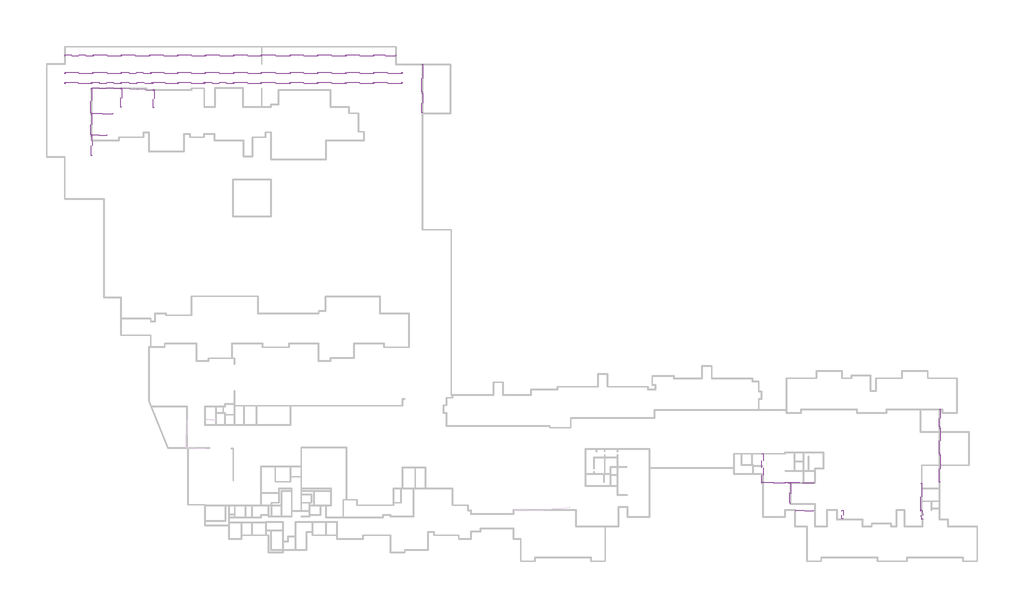
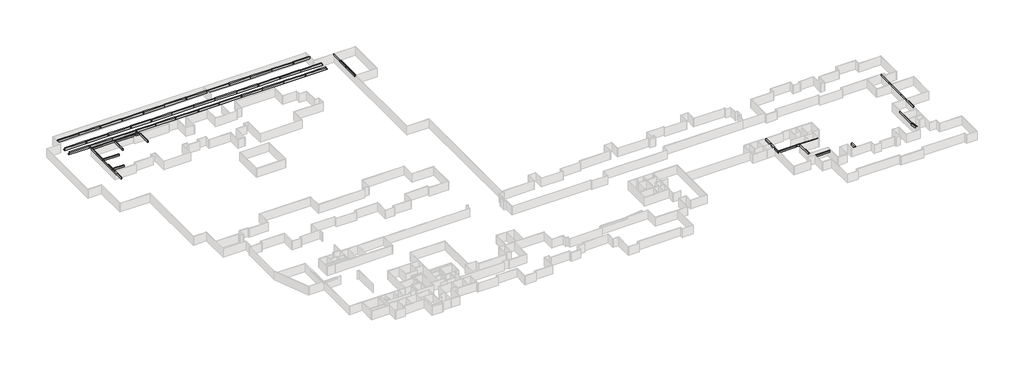
# One storey, part 8 of 8: 58 beams.
"""IFC4 building model written with IfcOpenShell, lengths in millimetres."""

from ifc_helpers import new_model, si_unit, frame, origin, place, context, project, spatial, polyline, outline, extrude, faceted_brep, element, save

model = new_model("IFC4")

# Units and contexts
model_context = context("Model", 3, world=origin())
ifc_project = project(units=[si_unit("LENGTHUNIT", "METRE", prefix="MILLI")], contexts=[model_context])

# Site, building, storey
site = spatial("IfcSite", under=ifc_project)
building = spatial("IfcBuilding", under=site)
storey = spatial("IfcBuildingStorey", under=building, Name="户型图", Elevation=0.0)

# Beams
placement = place(None, origin())
element("IfcBeam", 1, ObjectType="混凝土 - 矩形梁 : KL_beam", at=placement, inside=storey, context=model_context, shape_type="Brep", body=[
    faceted_brep([(69846.6115888, 146493.9951293, 3300.0), (69823.484619, 146214.2806226, 3300.0), (69695.5125279, 146193.9951293, 3300.0), (69833.6976621, 146193.9951293, 3300.0), (77972.7452463, 146193.9951293, 3300.0), (77972.7452463, 146493.9951293, 3300.0), (69695.5125279, 146193.9951293, 2700.0), (69833.6976621, 146193.9951293, 2700.0), (77972.7452463, 146193.9951293, 2700.0), (69823.484619, 146214.2806226, 2700.0), (69846.6115888, 146493.9951293, 2700.0), (77972.7452463, 146493.9951293, 2700.0)], [[[0, 1, 2, 3, 4, 5]], [[2, 6, 7, 8, 4, 3]], [[9, 10, 11, 8, 7, 6]], [[10, 0, 5, 11]], [[9, 1, 0, 10]], [[1, 9, 6, 2]], [[5, 4, 8, 11]]]),
])
element("IfcBeam", 2, ObjectType="混凝土 - 矩形梁 : KL_beam", at=placement, inside=storey, context=model_context, shape_type="SweptSolid", body=[
    extrude(outline(polyline([(69533.6976621, 146168.3450494), (69695.5125279, 146193.9951293), (69833.6976621, 146193.9951293), (69833.6976621, 139317.045189), (69533.6976621, 139317.045189), (69533.6976621, 146168.3450494)])), frame((0.0, 0.0, 2700.0), z_axis=(0.0, 0.0, 1.0), x_axis=(1.0, 0.0, 0.0)), (0.0, 0.0, 1.0), 600.0),
])
element("IfcBeam", 3, ObjectType="混凝土 - 矩形梁 : KL_beam", at=placement, inside=storey, context=model_context, shape_type="SweptSolid", body=[
    extrude(outline(polyline([(75683.6976621, 139317.045189), (75683.6976621, 139017.045189), (69858.8476291, 139017.045189), (69858.8476291, 139317.045189), (75683.6976621, 139317.045189)])), frame((0.0, 0.0, 2700.0), z_axis=(0.0, 0.0, 1.0), x_axis=(1.0, 0.0, 0.0)), (0.0, 0.0, 1.0), 600.0),
])
element("IfcBeam", 4, ObjectType="混凝土 - 矩形梁 : KL_beam", at=placement, inside=storey, context=model_context, shape_type="Brep", body=[
    faceted_brep([(78272.7452463, 140994.6198884, 3300.0), (77972.7452463, 140994.6198884, 3300.0), (77972.7452463, 140994.6198884, 2700.0), (78272.7452463, 140994.6198884, 2700.0), (78272.7452463, 146185.5002249, 3300.0), (78272.7452463, 146193.9951293, 3300.0), (77972.7452463, 146193.9951293, 3300.0), (77972.7452463, 146193.9951293, 2700.0), (78272.7452463, 146193.9951293, 2700.0), (78272.7452463, 146185.5002249, 2700.0)], [[[0, 1, 2, 3]], [[1, 0, 4, 5, 6]], [[2, 1, 6, 7]], [[3, 2, 7, 8, 9]], [[0, 3, 9, 8, 5, 4]], [[6, 5, 8, 7]]]),
])
element("IfcBeam", 5, ObjectType="混凝土 - 矩形梁 : KL_beam", at=placement, inside=storey, context=model_context, shape_type="Brep", body=[
    faceted_brep([(87344.6832098, 140893.8703738, 3300.0), (87044.6832098, 140893.8703738, 3300.0), (87044.6832098, 140893.8703738, 2700.0), (87344.6832098, 140893.8703738, 2700.0), (87344.6832098, 145855.8003854, 3300.0), (87044.6832098, 145832.1898733, 3300.0), (87044.6832098, 145702.0347295, 3300.0), (87044.6832098, 145832.1898733, 2700.0), (87044.6832098, 145702.0347295, 2700.0), (87344.6832098, 145855.8003854, 2700.0)], [[[0, 1, 2, 3]], [[1, 0, 4, 5, 6]], [[2, 1, 6, 5, 7, 8]], [[3, 2, 8, 7, 9]], [[0, 3, 9, 4]], [[4, 9, 7, 5]]]),
])
element("IfcBeam", 6, ObjectType="混凝土 - 矩形梁 : KL_beam", at=placement, inside=storey, context=model_context, shape_type="Brep", body=[
    faceted_brep([(78272.7452463, 146485.9555292, 3300.0), (78272.7452463, 146193.9951293, 3300.0), (78272.7452463, 146185.5002249, 3300.0), (87044.6832098, 145702.0347295, 3300.0), (87044.6832098, 145832.1898733, 3300.0), (87017.4727846, 146003.9897368, 3300.0), (78272.7452463, 146185.5002249, 2700.0), (87044.6832098, 145702.0347295, 2700.0), (78272.7452463, 146193.9951293, 2700.0), (78272.7452463, 146485.9555292, 2700.0), (87017.4727846, 146003.9897368, 2700.0), (87044.6832098, 145832.1898733, 2700.0)], [[[0, 1, 2, 3, 4, 5]], [[2, 6, 7, 3]], [[6, 8, 9, 10, 11, 7]], [[9, 0, 5, 10]], [[0, 9, 8, 6, 2, 1]], [[5, 4, 11, 10]], [[4, 3, 7, 11]]]),
])
element("IfcBeam", 7, ObjectType="混凝土 - 矩形梁 : KL_beam", at=placement, inside=storey, context=model_context, shape_type="Brep", body=[
    faceted_brep([(73982.1511869, 133204.2446453, 3300.0), (73982.1511869, 132904.2446453, 3300.0), (73982.1511869, 132904.2446453, 2700.0), (73982.1511869, 133204.2446453, 2700.0), (69833.6976621, 133204.2446453, 3300.0), (69833.6976621, 132904.2446453, 3300.0), (69835.8783333, 132904.2446453, 3300.0), (69833.6976621, 132904.2446453, 2700.0), (69835.8783333, 132904.2446453, 2700.0), (69833.6976621, 133204.2446453, 2700.0)], [[[0, 1, 2, 3]], [[1, 0, 4, 5, 6]], [[2, 1, 6, 5, 7, 8]], [[3, 2, 8, 7, 9]], [[0, 3, 9, 4]], [[5, 4, 9, 7]]]),
])
element("IfcBeam", 8, ObjectType="混凝土 - 矩形梁 : KL_beam", at=placement, inside=storey, context=model_context, shape_type="Brep", body=[
    faceted_brep([(258434.4881621, 35441.452007, 3300.0), (258434.4881621, 35141.452007, 3300.0), (264873.3530817, 35141.452007, 3300.0), (264873.3530817, 35441.452007, 3300.0), (258734.4881621, 35441.452007, 3300.0), (258434.4881621, 35441.452007, 2700.0), (264873.3530817, 35441.452007, 2700.0), (258734.4881621, 35441.452007, 2700.0), (258434.4881621, 35141.452007, 2700.0), (264873.3530817, 35141.452007, 2700.0)], [[[0, 1, 2, 3, 4]], [[5, 0, 4, 3, 6, 7]], [[8, 5, 7, 6, 9]], [[1, 8, 9, 2]], [[3, 2, 9, 6]], [[1, 0, 5, 8]]]),
])
element("IfcBeam", 9, ObjectType="混凝土 - 矩形梁 : KL_beam", at=placement, inside=storey, context=model_context, shape_type="SweptSolid", body=[
    extrude(outline(polyline([(258434.4881621, 43489.0128116), (258588.4160503, 43497.0798304), (258734.4881621, 43497.0798304), (258734.4881621, 35441.452007), (258434.4881621, 35441.452007), (258434.4881621, 43489.0128116)])), frame((0.0, 0.0, 2700.0), z_axis=(0.0, 0.0, 1.0), x_axis=(1.0, 0.0, 0.0)), (0.0, 0.0, 1.0), 600.0),
])
element("IfcBeam", 10, ObjectType="混凝土 - 矩形梁 : KL_beam", at=placement, inside=storey, context=model_context, shape_type="SweptSolid", body=[
    extrude(outline(polyline([(308273.5691593, 50816.8475615), (308573.5691593, 50816.8475615), (308573.5691593, 43416.8475615), (308273.5691593, 43416.8475615), (308273.5691593, 50816.8475615)])), frame((0.0, 0.0, 2700.0), z_axis=(0.0, 0.0, 1.0), x_axis=(1.0, 0.0, 0.0)), (0.0, 0.0, 1.0), 600.0),
])
element("IfcBeam", 11, ObjectType="混凝土 - 矩形梁 : KL_beam", at=placement, inside=storey, context=model_context, shape_type="SweptSolid", body=[
    extrude(outline(polyline([(308273.5691593, 43116.8475615), (308573.5691593, 43116.8475615), (308573.5691593, 35416.8475615), (308273.5691593, 35416.8475615), (308273.5691593, 43116.8475615)])), frame((0.0, 0.0, 2700.0), z_axis=(0.0, 0.0, 1.0), x_axis=(1.0, 0.0, 0.0)), (0.0, 0.0, 1.0), 600.0),
])
element("IfcBeam", 12, ObjectType="混凝土 - 矩形梁 : KL_beam", at=placement, inside=storey, context=model_context, shape_type="SweptSolid", body=[
    extrude(outline(polyline([(308273.5691593, 55914.1029719), (308573.5691593, 55914.1029719), (308573.5691593, 51116.8475615), (308273.5691593, 51116.8475615), (308273.5691593, 55914.1029719)])), frame((0.0, 0.0, 2700.0), z_axis=(0.0, 0.0, 1.0), x_axis=(1.0, 0.0, 0.0)), (0.0, 0.0, 1.0), 600.0),
])
element("IfcBeam", 13, ObjectType="混凝土 - 矩形梁 : KL_beam", at=placement, inside=storey, context=model_context, shape_type="SweptSolid", body=[
    extrude(outline(polyline([(162705.5468539, 144918.3398855), (163005.5468539, 144918.3398855), (163005.5468539, 139418.3398855), (162705.5468539, 139418.3398855), (162705.5468539, 144918.3398855)])), frame((0.0, 0.0, 2700.0), z_axis=(0.0, 0.0, 1.0), x_axis=(1.0, 0.0, 0.0)), (0.0, 0.0, 1.0), 600.0),
])
element("IfcBeam", 14, ObjectType="混凝土 - 矩形梁 : KL_beam", at=placement, inside=storey, context=model_context, shape_type="SweptSolid", body=[
    extrude(outline(polyline([(162705.5468539, 153068.3398855), (163005.5468539, 153068.3398855), (163005.5468539, 145218.3398855), (162705.5468539, 145218.3398855), (162705.5468539, 153068.3398855)])), frame((0.0, 0.0, 2700.0), z_axis=(0.0, 0.0, 1.0), x_axis=(1.0, 0.0, 0.0)), (0.0, 0.0, 1.0), 600.0),
])
element("IfcBeam", 15, ObjectType="混凝土 - 矩形梁 : KL_beam", at=placement, inside=storey, context=model_context, shape_type="SweptSolid", body=[
    extrude(outline(polyline([(69833.6976621, 133204.2446453), (69533.6976621, 133204.2446453), (69533.6976621, 139017.045189), (69833.6976621, 139017.045189), (69833.6976621, 133204.2446453)])), frame((0.0, 0.0, 2700.0), z_axis=(0.0, 0.0, 1.0), x_axis=(1.0, 0.0, 0.0)), (0.0, 0.0, 1.0), 600.0),
])
element("IfcBeam", 16, ObjectType="混凝土 - 矩形梁 : KL_beam", at=placement, inside=storey, context=model_context, shape_type="Brep", body=[
    faceted_brep([(69835.8783333, 132904.2446453, 2700.0), (69835.8783333, 132904.2446453, 3300.0), (69916.2512738, 127335.802002, 3300.0), (69916.2512738, 127335.802002, 2700.0), (69535.8470854, 132904.2446453, 2700.0), (69535.8470854, 132904.2446453, 3300.0), (69833.6976621, 132904.2446453, 3300.0), (69833.6976621, 132904.2446453, 2700.0), (69616.2200259, 127335.802002, 3300.0), (69908.2779599, 127335.802002, 3300.0), (69616.2200259, 127335.802002, 2700.0), (69908.2779599, 127335.802002, 2700.0)], [[[0, 1, 2, 3]], [[4, 5, 6, 1, 0, 7]], [[1, 6, 5, 8, 9, 2]], [[5, 4, 10, 8]], [[4, 7, 0, 3, 11, 10]], [[3, 2, 9, 8, 10, 11]]]),
])
element("IfcBeam", 17, ObjectType="混凝土 - 矩形梁 : KL_beam", at=placement, inside=storey, context=model_context, shape_type="Brep", body=[
    faceted_brep([(272934.4881621, 35141.452007, 3300.0), (272934.4881621, 35416.8475615, 3300.0), (272934.4881621, 35441.452007, 3300.0), (265173.3530817, 35441.452007, 3300.0), (265173.3530817, 35141.452007, 3300.0), (266273.353082, 35141.452007, 3300.0), (266573.353082, 35141.452007, 3300.0), (272934.4881621, 35141.452007, 2700.0), (265173.3530817, 35141.452007, 2700.0), (266273.353082, 35141.452007, 2700.0), (266573.353082, 35141.452007, 2700.0), (272934.4881621, 35441.452007, 2700.0), (272934.4881621, 35416.8475615, 2700.0), (265173.3530817, 35441.452007, 2700.0)], [[[0, 1, 2, 3, 4, 5, 6]], [[7, 0, 6, 5, 4, 8, 9, 10]], [[11, 12, 7, 10, 9, 8, 13]], [[2, 11, 13, 3]], [[0, 7, 12, 11, 2, 1]], [[4, 3, 13, 8]]]),
])
element("IfcBeam", 18, ObjectType="混凝土 - 矩形梁 : KL_beam", at=placement, inside=storey, context=model_context, shape_type="SweptSolid", body=[
    extrude(outline(polyline([(272934.4881621, 27616.8475615), (272934.4881621, 27479.970861), (272905.7251232, 27316.8475615), (268088.7951021, 27316.8475615), (267861.5245326, 27616.8475615), (272934.4881621, 27616.8475615)])), frame((0.0, 0.0, 2700.0), z_axis=(0.0, 0.0, 1.0), x_axis=(1.0, 0.0, 0.0)), (0.0, 0.0, 1.0), 600.0),
])
element("IfcBeam", 19, ObjectType="混凝土 - 矩形梁 : KL_beam", at=placement, inside=storey, context=model_context, shape_type="SweptSolid", body=[
    extrude(outline(polyline([(266573.353082, 29317.2500198), (266273.353082, 29713.2537795), (266273.353082, 35141.452007), (266573.353082, 35141.452007), (266573.353082, 29317.2500198)])), frame((0.0, 0.0, 2700.0), z_axis=(0.0, 0.0, 1.0), x_axis=(1.0, 0.0, 0.0)), (0.0, 0.0, 1.0), 600.0),
])
element("IfcBeam", 20, ObjectType="混凝土 - 矩形梁 : KL_beam", at=placement, inside=storey, context=model_context, shape_type="SweptSolid", body=[
    extrude(outline(polyline([(303434.4881621, 27527.6742369), (303134.4881621, 27527.6742369), (303134.4881621, 35116.8475615), (303434.4881621, 35116.8475615), (303434.4881621, 27527.6742369)])), frame((0.0, 0.0, 2700.0), z_axis=(0.0, 0.0, 1.0), x_axis=(1.0, 0.0, 0.0)), (0.0, 0.0, 1.0), 600.0),
])
element("IfcBeam", 21, ObjectType="混凝土 - 矩形梁 : L_beam", at=placement, inside=storey, context=model_context, shape_type="SweptSolid", body=[
    extrude(outline(polyline([(3300.0, 62199.2726456), (2500.0, 62199.2726456), (2500.0, 70393.6976621), (2700.0, 70393.6976621), (2700.0, 70093.6976621), (3300.0, 70093.6976621), (3300.0, 62199.2726456)])), frame((0.0, 155366.9462381, 0.0), z_axis=(0.0, 1.0, 0.0), x_axis=(0.0, 0.0, 1.0)), (0.0, 0.0, 1.0), 400.0),
])
element("IfcBeam", 22, ObjectType="混凝土 - 矩形梁 : L_beam", at=placement, inside=storey, context=model_context, shape_type="Brep", body=[
    faceted_brep([(70393.6976621, 155766.9462381, 3300.0), (70393.6976621, 155366.9462381, 3300.0), (77972.7452463, 155366.9462381, 3300.0), (77972.7452463, 155766.9462381, 3300.0), (70393.6976621, 155366.9462381, 2700.0), (70393.6976621, 155366.9462381, 2500.0), (78272.7452463, 155366.9462381, 2500.0), (78272.7452463, 155366.9462381, 2700.0), (77972.7452463, 155366.9462381, 2700.0), (78272.7452463, 155766.9462381, 2500.0), (70393.6976621, 155766.9462381, 2500.0), (70393.6976621, 155766.9462381, 2700.0), (77972.7452463, 155766.9462381, 2700.0), (78272.7452463, 155766.9462381, 2700.0)], [[[0, 1, 2, 3]], [[1, 4, 5, 6, 7, 8, 2]], [[9, 6, 5, 10]], [[10, 11, 0, 3, 12, 13, 9]], [[6, 9, 13, 7]], [[1, 0, 11, 10, 5, 4]], [[8, 12, 3, 2]], [[12, 8, 7, 13]]]),
])
element("IfcBeam", 23, ObjectType="混凝土 - 矩形梁 : L_beam", at=placement, inside=storey, context=model_context, shape_type="Brep", body=[
    faceted_brep([(78272.7452463, 155766.9462381, 3300.0), (78272.7452463, 155366.9462381, 3300.0), (85892.7452463, 155366.9462381, 3300.0), (85892.7452463, 155766.9462381, 3300.0), (78272.7452463, 155366.9462381, 2700.0), (78272.7452463, 155366.9462381, 2500.0), (86192.7452463, 155366.9462381, 2500.0), (86192.7452463, 155366.9462381, 2700.0), (85892.7452463, 155366.9462381, 2700.0), (86192.7452463, 155766.9462381, 2500.0), (78272.7452463, 155766.9462381, 2500.0), (78272.7452463, 155766.9462381, 2700.0), (85892.7452463, 155766.9462381, 2700.0), (86192.7452463, 155766.9462381, 2700.0)], [[[0, 1, 2, 3]], [[1, 4, 5, 6, 7, 8, 2]], [[9, 6, 5, 10]], [[10, 11, 0, 3, 12, 13, 9]], [[6, 9, 13, 7]], [[1, 0, 11, 10, 5, 4]], [[8, 12, 3, 2]], [[12, 8, 7, 13]]]),
])
element("IfcBeam", 24, ObjectType="混凝土 - 矩形梁 : L_beam", at=placement, inside=storey, context=model_context, shape_type="Brep", body=[
    faceted_brep([(86192.7452463, 155766.9462381, 3300.0), (86192.7452463, 155366.9462381, 3300.0), (93782.8755148, 155366.9462381, 3300.0), (93782.8755148, 155766.9462381, 3300.0), (86192.7452463, 155366.9462381, 2700.0), (86192.7452463, 155366.9462381, 2500.0), (94082.8755148, 155366.9462381, 2500.0), (94082.8755148, 155366.9462381, 2700.0), (93782.8755148, 155366.9462381, 2700.0), (94082.8755148, 155766.9462381, 2500.0), (86192.7452463, 155766.9462381, 2500.0), (86192.7452463, 155766.9462381, 2700.0), (93782.8755148, 155766.9462381, 2700.0), (94082.8755148, 155766.9462381, 2700.0)], [[[0, 1, 2, 3]], [[1, 4, 5, 6, 7, 8, 2]], [[9, 6, 5, 10]], [[10, 11, 0, 3, 12, 13, 9]], [[6, 9, 13, 7]], [[1, 0, 11, 10, 5, 4]], [[8, 12, 3, 2]], [[12, 8, 7, 13]]]),
])
element("IfcBeam", 25, ObjectType="混凝土 - 矩形梁 : L_beam", at=placement, inside=storey, context=model_context, shape_type="Brep", body=[
    faceted_brep([(94082.8755148, 155766.9462381, 3300.0), (94082.8755148, 155366.9462381, 3300.0), (101642.8755148, 155366.9462381, 3300.0), (101642.8755148, 155766.9462381, 3300.0), (94082.8755148, 155366.9462381, 2700.0), (94082.8755148, 155366.9462381, 2500.0), (101942.8755148, 155366.9462381, 2500.0), (101942.8755148, 155366.9462381, 2700.0), (101642.8755148, 155366.9462381, 2700.0), (101942.8755148, 155766.9462381, 2500.0), (94082.8755148, 155766.9462381, 2500.0), (94082.8755148, 155766.9462381, 2700.0), (101642.8755148, 155766.9462381, 2700.0), (101942.8755148, 155766.9462381, 2700.0)], [[[0, 1, 2, 3]], [[1, 4, 5, 6, 7, 8, 2]], [[9, 6, 5, 10]], [[10, 11, 0, 3, 12, 13, 9]], [[6, 9, 13, 7]], [[1, 0, 11, 10, 5, 4]], [[8, 12, 3, 2]], [[12, 8, 7, 13]]]),
])
element("IfcBeam", 26, ObjectType="混凝土 - 矩形梁 : L_beam", at=placement, inside=storey, context=model_context, shape_type="Brep", body=[
    faceted_brep([(101942.8755148, 155766.9462381, 3300.0), (101942.8755148, 155366.9462381, 3300.0), (109588.82396, 155366.9462381, 3300.0), (109588.82396, 155766.9462381, 3300.0), (101942.8755148, 155366.9462381, 2700.0), (101942.8755148, 155366.9462381, 2500.0), (109888.82396, 155366.9462381, 2500.0), (109888.82396, 155366.9462381, 2700.0), (109588.82396, 155366.9462381, 2700.0), (109888.82396, 155766.9462381, 2500.0), (101942.8755148, 155766.9462381, 2500.0), (101942.8755148, 155766.9462381, 2700.0), (109588.82396, 155766.9462381, 2700.0), (109888.82396, 155766.9462381, 2700.0)], [[[0, 1, 2, 3]], [[1, 4, 5, 6, 7, 8, 2]], [[9, 6, 5, 10]], [[10, 11, 0, 3, 12, 13, 9]], [[6, 9, 13, 7]], [[1, 0, 11, 10, 5, 4]], [[8, 12, 3, 2]], [[12, 8, 7, 13]]]),
])
element("IfcBeam", 27, ObjectType="混凝土 - 矩形梁 : L_beam", at=placement, inside=storey, context=model_context, shape_type="Brep", body=[
    faceted_brep([(109888.82396, 155766.9462381, 3300.0), (109888.82396, 155366.9462381, 3300.0), (117373.8474258, 155366.9462381, 3300.0), (117373.8474258, 155766.9462381, 3300.0), (109888.82396, 155366.9462381, 2700.0), (109888.82396, 155366.9462381, 2500.0), (117673.8474258, 155366.9462381, 2500.0), (117673.8474258, 155366.9462381, 2700.0), (117373.8474258, 155366.9462381, 2700.0), (117673.8474258, 155766.9462381, 2500.0), (109888.82396, 155766.9462381, 2500.0), (109888.82396, 155766.9462381, 2700.0), (117373.8474258, 155766.9462381, 2700.0), (117673.8474258, 155766.9462381, 2700.0)], [[[0, 1, 2, 3]], [[1, 4, 5, 6, 7, 8, 2]], [[9, 6, 5, 10]], [[10, 11, 0, 3, 12, 13, 9]], [[6, 9, 13, 7]], [[1, 0, 11, 10, 5, 4]], [[8, 12, 3, 2]], [[12, 8, 7, 13]]]),
])
element("IfcBeam", 28, ObjectType="混凝土 - 矩形梁 : L_beam", at=placement, inside=storey, context=model_context, shape_type="Brep", body=[
    faceted_brep([(117673.8474258, 155766.9462381, 3300.0), (117673.8474258, 155366.9462381, 3300.0), (125442.6046447, 155366.9462381, 3300.0), (125442.6046447, 155766.9462381, 3300.0), (117673.8474258, 155366.9462381, 2700.0), (117673.8474258, 155366.9462381, 2500.0), (125742.6046447, 155366.9462381, 2500.0), (125742.6046447, 155366.9462381, 2700.0), (125442.6046447, 155366.9462381, 2700.0), (125742.6046447, 155766.9462381, 2500.0), (117673.8474258, 155766.9462381, 2500.0), (117673.8474258, 155766.9462381, 2700.0), (125442.6046447, 155766.9462381, 2700.0), (125742.6046447, 155766.9462381, 2700.0)], [[[0, 1, 2, 3]], [[1, 4, 5, 6, 7, 8, 2]], [[9, 6, 5, 10]], [[10, 11, 0, 3, 12, 13, 9]], [[6, 9, 13, 7]], [[1, 0, 11, 10, 5, 4]], [[8, 12, 3, 2]], [[12, 8, 7, 13]]]),
])
element("IfcBeam", 29, ObjectType="混凝土 - 矩形梁 : L_beam", at=placement, inside=storey, context=model_context, shape_type="Brep", body=[
    faceted_brep([(125742.6046447, 155766.9462381, 3300.0), (125742.6046447, 155366.9462381, 3300.0), (133282.6046447, 155366.9462381, 3300.0), (133282.6046447, 155766.9462381, 3300.0), (125742.6046447, 155366.9462381, 2700.0), (125742.6046447, 155366.9462381, 2500.0), (133582.6046447, 155366.9462381, 2500.0), (133582.6046447, 155366.9462381, 2700.0), (133282.6046447, 155366.9462381, 2700.0), (133582.6046447, 155766.9462381, 2500.0), (125742.6046447, 155766.9462381, 2500.0), (125742.6046447, 155766.9462381, 2700.0), (133282.6046447, 155766.9462381, 2700.0), (133582.6046447, 155766.9462381, 2700.0)], [[[0, 1, 2, 3]], [[1, 4, 5, 6, 7, 8, 2]], [[9, 6, 5, 10]], [[10, 11, 0, 3, 12, 13, 9]], [[6, 9, 13, 7]], [[1, 0, 11, 10, 5, 4]], [[8, 12, 3, 2]], [[12, 8, 7, 13]]]),
])
element("IfcBeam", 30, ObjectType="混凝土 - 矩形梁 : L_beam", at=placement, inside=storey, context=model_context, shape_type="Brep", body=[
    faceted_brep([(133582.6046447, 155766.9462381, 3300.0), (133582.6046447, 155366.9462381, 3300.0), (141183.4366403, 155366.9462381, 3300.0), (141183.4366403, 155766.9462381, 3300.0), (133582.6046447, 155366.9462381, 2700.0), (133582.6046447, 155366.9462381, 2500.0), (141483.4366403, 155366.9462381, 2500.0), (141483.4366403, 155366.9462381, 2700.0), (141183.4366403, 155366.9462381, 2700.0), (141483.4366403, 155766.9462381, 2500.0), (133582.6046447, 155766.9462381, 2500.0), (133582.6046447, 155766.9462381, 2700.0), (141183.4366403, 155766.9462381, 2700.0), (141483.4366403, 155766.9462381, 2700.0)], [[[0, 1, 2, 3]], [[1, 4, 5, 6, 7, 8, 2]], [[9, 6, 5, 10]], [[10, 11, 0, 3, 12, 13, 9]], [[6, 9, 13, 7]], [[1, 0, 11, 10, 5, 4]], [[8, 12, 3, 2]], [[12, 8, 7, 13]]]),
])
element("IfcBeam", 31, ObjectType="混凝土 - 矩形梁 : L_beam", at=placement, inside=storey, context=model_context, shape_type="Brep", body=[
    faceted_brep([(141483.4366403, 155766.9462381, 3300.0), (141483.4366403, 155366.9462381, 3300.0), (149003.4366403, 155366.9462381, 3300.0), (149003.4366403, 155766.9462381, 3300.0), (141483.4366403, 155366.9462381, 2700.0), (141483.4366403, 155366.9462381, 2500.0), (149303.4366403, 155366.9462381, 2500.0), (149303.4366403, 155366.9462381, 2700.0), (149003.4366403, 155366.9462381, 2700.0), (149303.4366403, 155766.9462381, 2500.0), (141483.4366403, 155766.9462381, 2500.0), (141483.4366403, 155766.9462381, 2700.0), (149003.4366403, 155766.9462381, 2700.0), (149303.4366403, 155766.9462381, 2700.0)], [[[0, 1, 2, 3]], [[1, 4, 5, 6, 7, 8, 2]], [[9, 6, 5, 10]], [[10, 11, 0, 3, 12, 13, 9]], [[6, 9, 13, 7]], [[1, 0, 11, 10, 5, 4]], [[8, 12, 3, 2]], [[12, 8, 7, 13]]]),
])
element("IfcBeam", 32, ObjectType="混凝土 - 矩形梁 : L_beam", at=placement, inside=storey, context=model_context, shape_type="Brep", body=[
    faceted_brep([(155398.6421347, 155766.9462381, 3300.0), (155398.6421347, 155366.9462381, 3300.0), (155398.6421347, 155366.9462381, 2500.0), (155398.6421347, 155766.9462381, 2500.0), (149303.4366403, 155766.9462381, 3300.0), (149303.4366403, 155366.9462381, 3300.0), (149303.4366403, 155366.9462381, 2700.0), (149303.4366403, 155366.9462381, 2500.0), (149303.4366403, 155766.9462381, 2500.0), (149303.4366403, 155766.9462381, 2700.0)], [[[0, 1, 2, 3]], [[1, 0, 4, 5]], [[2, 1, 5, 6, 7]], [[3, 2, 7, 8]], [[0, 3, 8, 9, 4]], [[5, 4, 9, 8, 7, 6]]]),
])
element("IfcBeam", 33, ObjectType="混凝土 - 矩形梁 : L_beam", at=placement, inside=storey, context=model_context, shape_type="SweptSolid", body=[
    extrude(outline(polyline([(2500.0, 149003.4366403), (2500.0, 157205.5468539), (2700.0, 157205.5468539), (2700.0, 156905.5468539), (3300.0, 156905.5468539), (3300.0, 149303.4366403), (2700.0, 149303.4366403), (2700.0, 149003.4366403), (2500.0, 149003.4366403)])), frame((0.0, 150406.6496336, 0.0), z_axis=(0.0, 1.0, 0.0), x_axis=(0.0, 0.0, 1.0)), (0.0, 0.0, 1.0), 400.0),
])
element("IfcBeam", 34, ObjectType="混凝土 - 矩形梁 : L_beam", at=placement, inside=storey, context=model_context, shape_type="SweptSolid", body=[
    extrude(outline(polyline([(2500.0, 149003.4366403), (2500.0, 157205.5468539), (2700.0, 157205.5468539), (2700.0, 156905.5468539), (3300.0, 156905.5468539), (3300.0, 149303.4366403), (2700.0, 149303.4366403), (2700.0, 149003.4366403), (2500.0, 149003.4366403)])), frame((0.0, 147654.2446479, 0.0), z_axis=(0.0, 1.0, 0.0), x_axis=(0.0, 0.0, 1.0)), (0.0, 0.0, 1.0), 400.0),
])
element("IfcBeam", 35, ObjectType="混凝土 - 矩形梁 : L_beam", at=placement, inside=storey, context=model_context, shape_type="Brep", body=[
    faceted_brep([(281284.4881621, 25107.4835121, 3300.0), (280884.4881621, 25107.4835121, 3300.0), (280884.4881621, 25107.4835121, 2500.0), (281284.4881621, 25107.4835121, 2500.0), (281284.4881621, 27316.8475615, 3300.0), (281284.4881621, 27616.8475615, 3300.0), (281234.4881621, 27616.8475615, 3300.0), (280934.4881621, 27616.8475615, 3300.0), (280884.4881621, 27616.8475615, 3300.0), (280884.4881621, 27316.8475615, 3300.0), (280884.4881621, 27616.8475615, 2700.0), (280884.4881621, 27616.8475615, 2500.0), (281284.4881621, 27616.8475615, 2500.0), (281284.4881621, 27616.8475615, 2700.0)], [[[0, 1, 2, 3]], [[1, 0, 4, 5, 6, 7, 8, 9]], [[2, 1, 9, 8, 10, 11]], [[3, 2, 11, 12]], [[0, 3, 12, 13, 5, 4]], [[8, 7, 6, 5, 13, 12, 11, 10]]]),
])
element("IfcBeam", 36, ObjectType="混凝土 - 矩形梁 : L_beam", at=placement, inside=storey, context=model_context, shape_type="Brep", body=[
    faceted_brep([(303796.8162849, 25034.1829046, 3300.0), (303400.2834394, 24981.631002, 3300.0), (303400.2834394, 24981.631002, 2500.0), (303796.8162849, 25034.1829046, 2500.0), (303506.116172, 27227.6742369, 3300.0), (303466.3576224, 27527.6742369, 3300.0), (303434.4881621, 27527.6742369, 3300.0), (303134.4881621, 27527.6742369, 3300.0), (303062.8601522, 27527.6742369, 3300.0), (303102.6187017, 27227.6742369, 3300.0), (303062.8601522, 27527.6742369, 2700.0), (303062.8601522, 27527.6742369, 2500.0), (303466.3576224, 27527.6742369, 2500.0), (303466.3576224, 27527.6742369, 2700.0)], [[[0, 1, 2, 3]], [[1, 0, 4, 5, 6, 7, 8, 9]], [[2, 1, 9, 8, 10, 11]], [[3, 2, 11, 12]], [[0, 3, 12, 13, 5, 4]], [[8, 7, 6, 5, 13, 12, 11, 10]]]),
])
element("IfcBeam", 37, ObjectType="混凝土 - 矩形梁 : L_beam", at=placement, inside=storey, context=model_context, shape_type="Brep", body=[
    faceted_brep([(141483.4366403, 150806.6496336, 3300.0), (141483.4366403, 150406.6496336, 3300.0), (149003.4366403, 150406.6496336, 3300.0), (149003.4366403, 150806.6496336, 3300.0), (141183.4366403, 150806.6496336, 2500.0), (141183.4366403, 150806.6496336, 2700.0), (141483.4366403, 150806.6496336, 2700.0), (149003.4366403, 150806.6496336, 2700.0), (149003.4366403, 150806.6496336, 2500.0), (141183.4366403, 150406.6496336, 2500.0), (149003.4366403, 150406.6496336, 2500.0), (141183.4366403, 150406.6496336, 2700.0), (149003.4366403, 150406.6496336, 2700.0), (141483.4366403, 150406.6496336, 2700.0)], [[[0, 1, 2, 3]], [[4, 5, 6, 0, 3, 7, 8]], [[9, 4, 8, 10]], [[11, 9, 10, 12, 2, 1, 13]], [[4, 9, 11, 5]], [[13, 6, 5, 11]], [[6, 13, 1, 0]], [[3, 2, 12, 10, 8, 7]]]),
])
element("IfcBeam", 38, ObjectType="混凝土 - 矩形梁 : L_beam", at=placement, inside=storey, context=model_context, shape_type="Brep", body=[
    faceted_brep([(141483.4366403, 148054.2446479, 3300.0), (141483.4366403, 147654.2446479, 3300.0), (149003.4366403, 147654.2446479, 3300.0), (149003.4366403, 148054.2446479, 3300.0), (141183.4366403, 148054.2446479, 2500.0), (141183.4366403, 148054.2446479, 2700.0), (141483.4366403, 148054.2446479, 2700.0), (149003.4366403, 148054.2446479, 2700.0), (149003.4366403, 148054.2446479, 2500.0), (141183.4366403, 147654.2446479, 2500.0), (149003.4366403, 147654.2446479, 2500.0), (141183.4366403, 147654.2446479, 2700.0), (149003.4366403, 147654.2446479, 2700.0), (141483.4366403, 147654.2446479, 2700.0)], [[[0, 1, 2, 3]], [[4, 5, 6, 0, 3, 7, 8]], [[9, 4, 8, 10]], [[11, 9, 10, 12, 2, 1, 13]], [[4, 9, 11, 5]], [[13, 6, 5, 11]], [[6, 13, 1, 0]], [[3, 2, 12, 10, 8, 7]]]),
])
element("IfcBeam", 39, ObjectType="混凝土 - 矩形梁 : L_beam", at=placement, inside=storey, context=model_context, shape_type="Brep", body=[
    faceted_brep([(133582.6046447, 150806.6496336, 3300.0), (133582.6046447, 150406.6496336, 3300.0), (141183.4366403, 150406.6496336, 3300.0), (141183.4366403, 150806.6496336, 3300.0), (133282.6046447, 150806.6496336, 2500.0), (133282.6046447, 150806.6496336, 2700.0), (133582.6046447, 150806.6496336, 2700.0), (141183.4366403, 150806.6496336, 2700.0), (141183.4366403, 150806.6496336, 2500.0), (133282.6046447, 150406.6496336, 2500.0), (141183.4366403, 150406.6496336, 2500.0), (133282.6046447, 150406.6496336, 2700.0), (141183.4366403, 150406.6496336, 2700.0), (133582.6046447, 150406.6496336, 2700.0)], [[[0, 1, 2, 3]], [[4, 5, 6, 0, 3, 7, 8]], [[9, 4, 8, 10]], [[11, 9, 10, 12, 2, 1, 13]], [[4, 9, 11, 5]], [[13, 6, 5, 11]], [[6, 13, 1, 0]], [[3, 2, 12, 10, 8, 7]]]),
])
element("IfcBeam", 40, ObjectType="混凝土 - 矩形梁 : L_beam", at=placement, inside=storey, context=model_context, shape_type="Brep", body=[
    faceted_brep([(133582.6046447, 148054.2446479, 3300.0), (133582.6046447, 147654.2446479, 3300.0), (141183.4366403, 147654.2446479, 3300.0), (141183.4366403, 148054.2446479, 3300.0), (133282.6046447, 148054.2446479, 2500.0), (133282.6046447, 148054.2446479, 2700.0), (133582.6046447, 148054.2446479, 2700.0), (141183.4366403, 148054.2446479, 2700.0), (141183.4366403, 148054.2446479, 2500.0), (133282.6046447, 147654.2446479, 2500.0), (141183.4366403, 147654.2446479, 2500.0), (133282.6046447, 147654.2446479, 2700.0), (141183.4366403, 147654.2446479, 2700.0), (133582.6046447, 147654.2446479, 2700.0)], [[[0, 1, 2, 3]], [[4, 5, 6, 0, 3, 7, 8]], [[9, 4, 8, 10]], [[11, 9, 10, 12, 2, 1, 13]], [[4, 9, 11, 5]], [[13, 6, 5, 11]], [[6, 13, 1, 0]], [[3, 2, 12, 10, 8, 7]]]),
])
element("IfcBeam", 41, ObjectType="混凝土 - 矩形梁 : L_beam", at=placement, inside=storey, context=model_context, shape_type="Brep", body=[
    faceted_brep([(125742.6046447, 150806.6496336, 3300.0), (125742.6046447, 150406.6496336, 3300.0), (133282.6046447, 150406.6496336, 3300.0), (133282.6046447, 150806.6496336, 3300.0), (125442.6046447, 150806.6496336, 2500.0), (125442.6046447, 150806.6496336, 2700.0), (125742.6046447, 150806.6496336, 2700.0), (133282.6046447, 150806.6496336, 2700.0), (133282.6046447, 150806.6496336, 2500.0), (125442.6046447, 150406.6496336, 2500.0), (133282.6046447, 150406.6496336, 2500.0), (125442.6046447, 150406.6496336, 2700.0), (133282.6046447, 150406.6496336, 2700.0), (125742.6046447, 150406.6496336, 2700.0)], [[[0, 1, 2, 3]], [[4, 5, 6, 0, 3, 7, 8]], [[9, 4, 8, 10]], [[11, 9, 10, 12, 2, 1, 13]], [[4, 9, 11, 5]], [[13, 6, 5, 11]], [[6, 13, 1, 0]], [[3, 2, 12, 10, 8, 7]]]),
])
element("IfcBeam", 42, ObjectType="混凝土 - 矩形梁 : L_beam", at=placement, inside=storey, context=model_context, shape_type="Brep", body=[
    faceted_brep([(125742.6046447, 148054.2446479, 3300.0), (125742.6046447, 147654.2446479, 3300.0), (133282.6046447, 147654.2446479, 3300.0), (133282.6046447, 148054.2446479, 3300.0), (125442.6046447, 148054.2446479, 2500.0), (125442.6046447, 148054.2446479, 2700.0), (125742.6046447, 148054.2446479, 2700.0), (133282.6046447, 148054.2446479, 2700.0), (133282.6046447, 148054.2446479, 2500.0), (125442.6046447, 147654.2446479, 2500.0), (133282.6046447, 147654.2446479, 2500.0), (125442.6046447, 147654.2446479, 2700.0), (133282.6046447, 147654.2446479, 2700.0), (125742.6046447, 147654.2446479, 2700.0)], [[[0, 1, 2, 3]], [[4, 5, 6, 0, 3, 7, 8]], [[9, 4, 8, 10]], [[11, 9, 10, 12, 2, 1, 13]], [[4, 9, 11, 5]], [[13, 6, 5, 11]], [[6, 13, 1, 0]], [[3, 2, 12, 10, 8, 7]]]),
])
element("IfcBeam", 43, ObjectType="混凝土 - 矩形梁 : L_beam", at=placement, inside=storey, context=model_context, shape_type="Brep", body=[
    faceted_brep([(117673.8474258, 150806.6496336, 3300.0), (117673.8474258, 150406.6496336, 3300.0), (125442.6046447, 150406.6496336, 3300.0), (125442.6046447, 150806.6496336, 3300.0), (117373.8474258, 150806.6496336, 2500.0), (117373.8474258, 150806.6496336, 2700.0), (117673.8474258, 150806.6496336, 2700.0), (125442.6046447, 150806.6496336, 2700.0), (125442.6046447, 150806.6496336, 2500.0), (117373.8474258, 150406.6496336, 2500.0), (125442.6046447, 150406.6496336, 2500.0), (117373.8474258, 150406.6496336, 2700.0), (125442.6046447, 150406.6496336, 2700.0), (117673.8474258, 150406.6496336, 2700.0)], [[[0, 1, 2, 3]], [[4, 5, 6, 0, 3, 7, 8]], [[9, 4, 8, 10]], [[11, 9, 10, 12, 2, 1, 13]], [[4, 9, 11, 5]], [[13, 6, 5, 11]], [[6, 13, 1, 0]], [[3, 2, 12, 10, 8, 7]]]),
])
element("IfcBeam", 44, ObjectType="混凝土 - 矩形梁 : L_beam", at=placement, inside=storey, context=model_context, shape_type="Brep", body=[
    faceted_brep([(117673.8474258, 148054.2446479, 3300.0), (117673.8474258, 147654.2446479, 3300.0), (125442.6046447, 147654.2446479, 3300.0), (125442.6046447, 148054.2446479, 3300.0), (117373.8474258, 148054.2446479, 2500.0), (117373.8474258, 148054.2446479, 2700.0), (117673.8474258, 148054.2446479, 2700.0), (125442.6046447, 148054.2446479, 2700.0), (125442.6046447, 148054.2446479, 2500.0), (117373.8474258, 147654.2446479, 2500.0), (125442.6046447, 147654.2446479, 2500.0), (117373.8474258, 147654.2446479, 2700.0), (125442.6046447, 147654.2446479, 2700.0), (117673.8474258, 147654.2446479, 2700.0)], [[[0, 1, 2, 3]], [[4, 5, 6, 0, 3, 7, 8]], [[9, 4, 8, 10]], [[11, 9, 10, 12, 2, 1, 13]], [[4, 9, 11, 5]], [[13, 6, 5, 11]], [[6, 13, 1, 0]], [[3, 2, 12, 10, 8, 7]]]),
])
element("IfcBeam", 45, ObjectType="混凝土 - 矩形梁 : L_beam", at=placement, inside=storey, context=model_context, shape_type="Brep", body=[
    faceted_brep([(109888.82396, 150806.6496336, 3300.0), (109888.82396, 150406.6496336, 3300.0), (117373.8474258, 150406.6496336, 3300.0), (117373.8474258, 150806.6496336, 3300.0), (109588.82396, 150806.6496336, 2500.0), (109588.82396, 150806.6496336, 2700.0), (109888.82396, 150806.6496336, 2700.0), (117373.8474258, 150806.6496336, 2700.0), (117373.8474258, 150806.6496336, 2500.0), (109588.82396, 150406.6496336, 2500.0), (117373.8474258, 150406.6496336, 2500.0), (109588.82396, 150406.6496336, 2700.0), (117373.8474258, 150406.6496336, 2700.0), (109888.82396, 150406.6496336, 2700.0)], [[[0, 1, 2, 3]], [[4, 5, 6, 0, 3, 7, 8]], [[9, 4, 8, 10]], [[11, 9, 10, 12, 2, 1, 13]], [[4, 9, 11, 5]], [[13, 6, 5, 11]], [[6, 13, 1, 0]], [[3, 2, 12, 10, 8, 7]]]),
])
element("IfcBeam", 46, ObjectType="混凝土 - 矩形梁 : L_beam", at=placement, inside=storey, context=model_context, shape_type="Brep", body=[
    faceted_brep([(109888.82396, 148054.2446479, 3300.0), (109888.82396, 147654.2446479, 3300.0), (117373.8474258, 147654.2446479, 3300.0), (117373.8474258, 148054.2446479, 3300.0), (109588.82396, 148054.2446479, 2500.0), (109588.82396, 148054.2446479, 2700.0), (109888.82396, 148054.2446479, 2700.0), (117373.8474258, 148054.2446479, 2700.0), (117373.8474258, 148054.2446479, 2500.0), (109588.82396, 147654.2446479, 2500.0), (117373.8474258, 147654.2446479, 2500.0), (109588.82396, 147654.2446479, 2700.0), (117373.8474258, 147654.2446479, 2700.0), (109888.82396, 147654.2446479, 2700.0)], [[[0, 1, 2, 3]], [[4, 5, 6, 0, 3, 7, 8]], [[9, 4, 8, 10]], [[11, 9, 10, 12, 2, 1, 13]], [[4, 9, 11, 5]], [[13, 6, 5, 11]], [[6, 13, 1, 0]], [[3, 2, 12, 10, 8, 7]]]),
])
element("IfcBeam", 47, ObjectType="混凝土 - 矩形梁 : L_beam", at=placement, inside=storey, context=model_context, shape_type="Brep", body=[
    faceted_brep([(101820.2809905, 150806.6496336, 3300.0), (101799.0194755, 150406.6496336, 3300.0), (109588.82396, 150406.6496336, 3300.0), (109588.82396, 150806.6496336, 3300.0), (101519.8574906, 150806.6496336, 2500.0), (101519.8574906, 150806.6496336, 2700.0), (101820.2809905, 150806.6496336, 2700.0), (109588.82396, 150806.6496336, 2700.0), (109588.82396, 150806.6496336, 2500.0), (101498.5959757, 150406.6496336, 2500.0), (109588.82396, 150406.6496336, 2500.0), (101498.5959757, 150406.6496336, 2700.0), (109588.82396, 150406.6496336, 2700.0), (101799.0194755, 150406.6496336, 2700.0)], [[[0, 1, 2, 3]], [[4, 5, 6, 0, 3, 7, 8]], [[9, 4, 8, 10]], [[11, 9, 10, 12, 2, 1, 13]], [[4, 9, 11, 5]], [[13, 6, 5, 11]], [[6, 13, 1, 0]], [[3, 2, 12, 10, 8, 7]]]),
])
element("IfcBeam", 48, ObjectType="混凝土 - 矩形梁 : L_beam", at=placement, inside=storey, context=model_context, shape_type="Brep", body=[
    faceted_brep([(101673.9802411, 148054.2446479, 3300.0), (101652.7187262, 147654.2446479, 3300.0), (109588.82396, 147654.2446479, 3300.0), (109588.82396, 148054.2446479, 3300.0), (101373.5567413, 148054.2446479, 2500.0), (101373.5567413, 148054.2446479, 2700.0), (101673.9802411, 148054.2446479, 2700.0), (109588.82396, 148054.2446479, 2700.0), (109588.82396, 148054.2446479, 2500.0), (101352.2952263, 147654.2446479, 2500.0), (109588.82396, 147654.2446479, 2500.0), (101352.2952263, 147654.2446479, 2700.0), (109588.82396, 147654.2446479, 2700.0), (101652.7187262, 147654.2446479, 2700.0)], [[[0, 1, 2, 3]], [[4, 5, 6, 0, 3, 7, 8]], [[9, 4, 8, 10]], [[11, 9, 10, 12, 2, 1, 13]], [[4, 9, 11, 5]], [[13, 6, 5, 11]], [[6, 13, 1, 0]], [[3, 2, 12, 10, 8, 7]]]),
])
element("IfcBeam", 49, ObjectType="混凝土 - 矩形梁 : L_beam", at=placement, inside=storey, context=model_context, shape_type="Brep", body=[
    faceted_brep([(94163.6477371, 150806.6496336, 3300.0), (94177.6160449, 150406.6496336, 3300.0), (101498.5959757, 150406.6496336, 3300.0), (101519.8574906, 150806.6496336, 3300.0), (93863.4648738, 150806.6496336, 2500.0), (93863.4648738, 150806.6496336, 2700.0), (94163.6477371, 150806.6496336, 2700.0), (101519.8574906, 150806.6496336, 2700.0), (101519.8574906, 150806.6496336, 2500.0), (93877.4331816, 150406.6496336, 2500.0), (101498.5959757, 150406.6496336, 2500.0), (93877.4331816, 150406.6496336, 2700.0), (101498.5959757, 150406.6496336, 2700.0), (94177.6160449, 150406.6496336, 2700.0)], [[[0, 1, 2, 3]], [[4, 5, 6, 0, 3, 7, 8]], [[9, 4, 8, 10]], [[11, 9, 10, 12, 2, 1, 13]], [[4, 9, 11, 5]], [[13, 6, 5, 11]], [[6, 13, 1, 0]], [[3, 2, 12, 10, 8, 7]]]),
])
element("IfcBeam", 50, ObjectType="混凝土 - 矩形梁 : L_beam", at=placement, inside=storey, context=model_context, shape_type="Brep", body=[
    faceted_brep([(94259.7638372, 148054.2446479, 3300.0), (94273.732145, 147654.2446479, 3300.0), (101352.2952263, 147654.2446479, 3300.0), (101373.5567413, 148054.2446479, 3300.0), (93959.5809739, 148054.2446479, 2500.0), (93959.5809739, 148054.2446479, 2700.0), (94259.7638372, 148054.2446479, 2700.0), (101373.5567413, 148054.2446479, 2700.0), (101373.5567413, 148054.2446479, 2500.0), (93973.5492817, 147654.2446479, 2500.0), (101352.2952263, 147654.2446479, 2500.0), (93973.5492817, 147654.2446479, 2700.0), (101352.2952263, 147654.2446479, 2700.0), (94273.732145, 147654.2446479, 2700.0)], [[[0, 1, 2, 3]], [[4, 5, 6, 0, 3, 7, 8]], [[9, 4, 8, 10]], [[11, 9, 10, 12, 2, 1, 13]], [[4, 9, 11, 5]], [[13, 6, 5, 11]], [[6, 13, 1, 0]], [[3, 2, 12, 10, 8, 7]]]),
])
element("IfcBeam", 51, ObjectType="混凝土 - 矩形梁 : L_beam", at=placement, inside=storey, context=model_context, shape_type="Brep", body=[
    faceted_brep([(86560.5457225, 150806.6496336, 3300.0), (86623.8994986, 150406.6496336, 3300.0), (93877.4331816, 150406.6496336, 3300.0), (93863.4648738, 150806.6496336, 3300.0), (86256.8061848, 150806.6496336, 2500.0), (86256.8061848, 150806.6496336, 2700.0), (86560.5457225, 150806.6496336, 2700.0), (93863.4648738, 150806.6496336, 2700.0), (93863.4648738, 150806.6496336, 2500.0), (86320.1599609, 150406.6496336, 2500.0), (93877.4331816, 150406.6496336, 2500.0), (86320.1599609, 150406.6496336, 2700.0), (93877.4331816, 150406.6496336, 2700.0), (86623.8994986, 150406.6496336, 2700.0)], [[[0, 1, 2, 3]], [[4, 5, 6, 0, 3, 7, 8]], [[9, 4, 8, 10]], [[11, 9, 10, 12, 2, 1, 13]], [[4, 9, 11, 5]], [[13, 6, 5, 11]], [[6, 13, 1, 0]], [[3, 2, 12, 10, 8, 7]]]),
])
element("IfcBeam", 52, ObjectType="混凝土 - 矩形梁 : L_beam", at=placement, inside=storey, context=model_context, shape_type="Brep", body=[
    faceted_brep([(86996.4838457, 148054.2446479, 3300.0), (87059.8376218, 147654.2446479, 3300.0), (93973.5492817, 147654.2446479, 3300.0), (93959.5809739, 148054.2446479, 3300.0), (86692.744308, 148054.2446479, 2500.0), (86692.744308, 148054.2446479, 2700.0), (86996.4838457, 148054.2446479, 2700.0), (93959.5809739, 148054.2446479, 2700.0), (93959.5809739, 148054.2446479, 2500.0), (86756.0980841, 147654.2446479, 2500.0), (93973.5492817, 147654.2446479, 2500.0), (86756.0980841, 147654.2446479, 2700.0), (93973.5492817, 147654.2446479, 2700.0), (87059.8376218, 147654.2446479, 2700.0)], [[[0, 1, 2, 3]], [[4, 5, 6, 0, 3, 7, 8]], [[9, 4, 8, 10]], [[11, 9, 10, 12, 2, 1, 13]], [[4, 9, 11, 5]], [[13, 6, 5, 11]], [[6, 13, 1, 0]], [[3, 2, 12, 10, 8, 7]]]),
])
element("IfcBeam", 53, ObjectType="混凝土 - 矩形梁 : L_beam", at=placement, inside=storey, context=model_context, shape_type="Brep", body=[
    faceted_brep([(78272.7452463, 150806.6496336, 3300.0), (78272.7452463, 150406.6496336, 3300.0), (86320.1599609, 150406.6496336, 3300.0), (86256.8061848, 150806.6496336, 3300.0), (77972.7452463, 150806.6496336, 2500.0), (77972.7452463, 150806.6496336, 2700.0), (78272.7452463, 150806.6496336, 2700.0), (86256.8061848, 150806.6496336, 2700.0), (86256.8061848, 150806.6496336, 2500.0), (77972.7452463, 150406.6496336, 2500.0), (86320.1599609, 150406.6496336, 2500.0), (77972.7452463, 150406.6496336, 2700.0), (86320.1599609, 150406.6496336, 2700.0), (78272.7452463, 150406.6496336, 2700.0)], [[[0, 1, 2, 3]], [[4, 5, 6, 0, 3, 7, 8]], [[9, 4, 8, 10]], [[11, 9, 10, 12, 2, 1, 13]], [[4, 9, 11, 5]], [[13, 6, 5, 11]], [[6, 13, 1, 0]], [[3, 2, 12, 10, 8, 7]]]),
])
element("IfcBeam", 54, ObjectType="混凝土 - 矩形梁 : L_beam", at=placement, inside=storey, context=model_context, shape_type="Brep", body=[
    faceted_brep([(78272.7452463, 148054.2446479, 3300.0), (78272.7452463, 147654.2446479, 3300.0), (86756.0980841, 147654.2446479, 3300.0), (86692.744308, 148054.2446479, 3300.0), (77972.7452463, 148054.2446479, 2500.0), (77972.7452463, 148054.2446479, 2700.0), (78272.7452463, 148054.2446479, 2700.0), (86692.744308, 148054.2446479, 2700.0), (86692.744308, 148054.2446479, 2500.0), (77972.7452463, 147654.2446479, 2500.0), (86756.0980841, 147654.2446479, 2500.0), (77972.7452463, 147654.2446479, 2700.0), (86756.0980841, 147654.2446479, 2700.0), (78272.7452463, 147654.2446479, 2700.0)], [[[0, 1, 2, 3]], [[4, 5, 6, 0, 3, 7, 8]], [[9, 4, 8, 10]], [[11, 9, 10, 12, 2, 1, 13]], [[4, 9, 11, 5]], [[13, 6, 5, 11]], [[6, 13, 1, 0]], [[3, 2, 12, 10, 8, 7]]]),
])
element("IfcBeam", 55, ObjectType="混凝土 - 矩形梁 : L_beam", at=placement, inside=storey, context=model_context, shape_type="Brep", body=[
    faceted_brep([(70203.1845508, 150806.6496336, 3300.0), (70170.1123015, 150406.6496336, 3300.0), (77972.7452463, 150406.6496336, 3300.0), (77972.7452463, 150806.6496336, 3300.0), (69902.1608844, 150806.6496336, 2500.0), (69902.1608844, 150806.6496336, 2700.0), (70203.1845508, 150806.6496336, 2700.0), (77972.7452463, 150806.6496336, 2700.0), (77972.7452463, 150806.6496336, 2500.0), (69869.0886352, 150406.6496336, 2500.0), (77972.7452463, 150406.6496336, 2500.0), (69869.0886352, 150406.6496336, 2700.0), (77972.7452463, 150406.6496336, 2700.0), (70170.1123015, 150406.6496336, 2700.0)], [[[0, 1, 2, 3]], [[4, 5, 6, 0, 3, 7, 8]], [[9, 4, 8, 10]], [[11, 9, 10, 12, 2, 1, 13]], [[4, 9, 11, 5]], [[13, 6, 5, 11]], [[6, 13, 1, 0]], [[3, 2, 12, 10, 8, 7]]]),
])
element("IfcBeam", 56, ObjectType="混凝土 - 矩形梁 : L_beam", at=placement, inside=storey, context=model_context, shape_type="Brep", body=[
    faceted_brep([(69975.6139913, 148054.2446479, 3300.0), (69942.541742, 147654.2446479, 3300.0), (77972.7452463, 147654.2446479, 3300.0), (77972.7452463, 148054.2446479, 3300.0), (69674.590325, 148054.2446479, 2500.0), (69674.590325, 148054.2446479, 2700.0), (69975.6139913, 148054.2446479, 2700.0), (77972.7452463, 148054.2446479, 2700.0), (77972.7452463, 148054.2446479, 2500.0), (69641.5180757, 147654.2446479, 2500.0), (77972.7452463, 147654.2446479, 2500.0), (69641.5180757, 147654.2446479, 2700.0), (77972.7452463, 147654.2446479, 2700.0), (69942.541742, 147654.2446479, 2700.0)], [[[0, 1, 2, 3]], [[4, 5, 6, 0, 3, 7, 8]], [[9, 4, 8, 10]], [[11, 9, 10, 12, 2, 1, 13]], [[4, 9, 11, 5]], [[13, 6, 5, 11]], [[6, 13, 1, 0]], [[3, 2, 12, 10, 8, 7]]]),
])
element("IfcBeam", 57, ObjectType="混凝土 - 矩形梁 : L_beam", at=placement, inside=storey, context=model_context, shape_type="Brep", body=[
    faceted_brep([(62408.8476291, 150806.6496336, 3300.0), (62408.8476291, 150406.6496336, 3300.0), (69869.0886352, 150406.6496336, 3300.0), (69902.1608844, 150806.6496336, 3300.0), (62108.8476291, 150806.6496336, 2500.0), (62108.8476291, 150806.6496336, 2700.0), (62408.8476291, 150806.6496336, 2700.0), (69902.1608844, 150806.6496336, 2700.0), (69902.1608844, 150806.6496336, 2500.0), (62108.8476291, 150406.6496336, 2500.0), (69869.0886352, 150406.6496336, 2500.0), (62108.8476291, 150406.6496336, 2700.0), (69869.0886352, 150406.6496336, 2700.0), (62408.8476291, 150406.6496336, 2700.0)], [[[0, 1, 2, 3]], [[4, 5, 6, 0, 3, 7, 8]], [[9, 4, 8, 10]], [[11, 9, 10, 12, 2, 1, 13]], [[4, 9, 11, 5]], [[13, 6, 5, 11]], [[6, 13, 1, 0]], [[3, 2, 12, 10, 8, 7]]]),
])
element("IfcBeam", 58, ObjectType="混凝土 - 矩形梁 : L_beam", at=placement, inside=storey, context=model_context, shape_type="Brep", body=[
    faceted_brep([(62408.8476291, 148054.2446479, 3300.0), (62408.8476291, 147654.2446479, 3300.0), (69641.5180757, 147654.2446479, 3300.0), (69674.590325, 148054.2446479, 3300.0), (62108.8476291, 148054.2446479, 2500.0), (62108.8476291, 148054.2446479, 2700.0), (62408.8476291, 148054.2446479, 2700.0), (69674.590325, 148054.2446479, 2700.0), (69674.590325, 148054.2446479, 2500.0), (62108.8476291, 147654.2446479, 2500.0), (69641.5180757, 147654.2446479, 2500.0), (62108.8476291, 147654.2446479, 2700.0), (69641.5180757, 147654.2446479, 2700.0), (62408.8476291, 147654.2446479, 2700.0)], [[[0, 1, 2, 3]], [[4, 5, 6, 0, 3, 7, 8]], [[9, 4, 8, 10]], [[11, 9, 10, 12, 2, 1, 13]], [[4, 9, 11, 5]], [[13, 6, 5, 11]], [[6, 13, 1, 0]], [[3, 2, 12, 10, 8, 7]]]),
])

save(model, "model.ifc")

# Revit data of these elements
# Type "混凝土 - 矩形梁 : KL_beam"
#   Length [instance default] = 1524 mm
#   b = 300 mm
#   h = 600 mm
#   Structural Material [instance default] = 混凝土 - 现场浇注混凝土
#   Assembly Code = ""
# Type "混凝土 - 矩形梁 : L_beam"
#   Length [instance default] = 1524 mm
#   b = 400 mm
#   h = 800 mm
#   Structural Material [instance default] = none
#   Assembly Code = ""
# Elements 1, 2, 3, 4, 5, 6, 7, 8, 9, 10, 11, 12, 13, 14, 15, 16, 17, 18, 19, 20 (IfcBeam, "混凝土 - 矩形梁 : KL_beam")
#   Comments = ""
#   Structural Material = none
#   Phase Created = 新构造
# Elements 21, 22, 23, 24, 25, 26, 27, 28, 29, 30, 31, 32, 33, 34, 35, 36, 37, 38, 39, 40, 41, 42, 43, 44, 45, 46, 47, 48, 49, 50, 51, 52, 53, 54, 55, 56, 57, 58 (IfcBeam, "混凝土 - 矩形梁 : L_beam")
#   Comments = ""
#   Structural Material = none
#   Phase Created = 新构造
# Materials
#   "混凝土 - 现场浇注混凝土": class "混凝土", colour RGB 192 192 192, transparency 0
